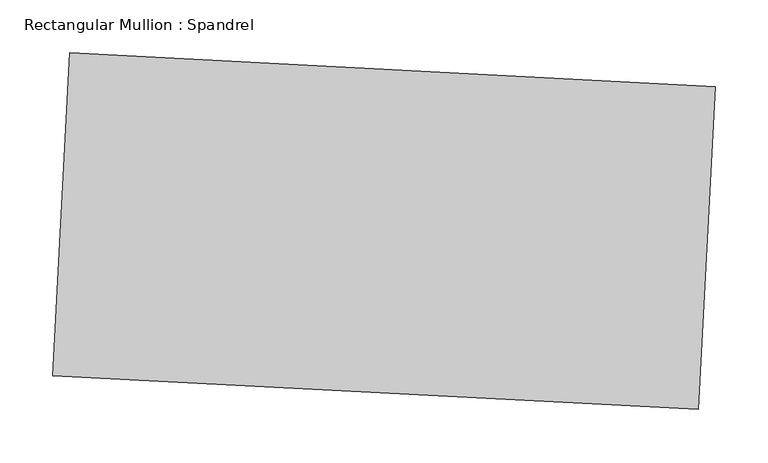
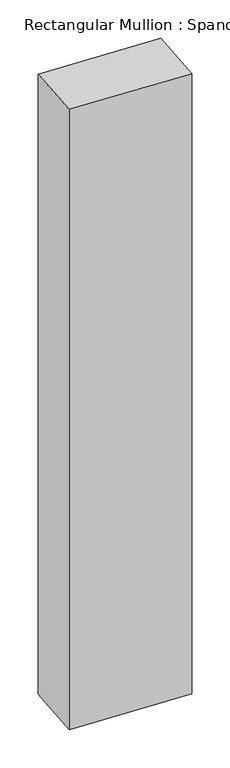
"""IFC4 building model written with IfcOpenShell, lengths in millimetres: member geometry, Rectangular Mullion : Spandrel."""

from ifc_helpers import new_model, si_unit, frame, origin, place, context, project, spatial, polyline, outline, extrude, source, transform, mapped, element, save


def rectangular_mullion_spandrel_e01d9ec2(model_context):
    return source(origin(), model_context, "Body", "SweptSolid", [
        extrude(outline(polyline([(312.3582819, 136.2391416), (296.4062825, -168.1431406), (-312.3582819, -136.2391416), (-296.4062825, 168.1431406), (312.3582819, 136.2391416)])), frame((0.0, 0.0, -3352.8), z_axis=(0.0, 0.0, 1.0), x_axis=(1.0, 0.0, 0.0)), (0.0, 0.0, 1.0), 3352.8),
    ])


if __name__ == "__main__":
    model = new_model("IFC4")
    model_context = context("Model", 3, world=origin())
    ifc_project = project(units=[si_unit("LENGTHUNIT", "METRE", prefix="MILLI")], contexts=[model_context])
    site = spatial("IfcSite", under=ifc_project)
    building = spatial("IfcBuilding", under=site)
    placement = place(None, origin())
    rectangular_mullion_spandrel_shape = rectangular_mullion_spandrel_e01d9ec2(model_context)
    element("IfcMember", 1, ObjectType="Rectangular Mullion : Spandrel", at=placement, inside=building, context=model_context, shape_type="MappedRepresentation", body=[
        mapped(rectangular_mullion_spandrel_shape, transform((0.0, 0.0, 0.0), x_axis=(1.0, 0.0, 0.0), y_axis=(0.0, 1.0, 0.0), z_axis=(0.0, 0.0, 1.0))),
    ])
    save(model, "model.ifc")

# Revit data of these elements
# Type "Rectangular Mullion : Spandrel"
#   built-in parameter 1007304 = 1 (stored number, unit not read)
#   built-in parameter 1007301 = 1 (stored number, unit not read)
#   built-in parameter 1007300 = 1 (stored number, unit not read)
# Element 1 (IfcMember, "Rectangular Mullion : Spandrel")
#   Materials on its faces: "Aluminum"
# Materials
#   "Aluminum": class "Metal", colour RGB 247 247 247, transparency 0, Description = "Aluminum 6061", Cost = 0
